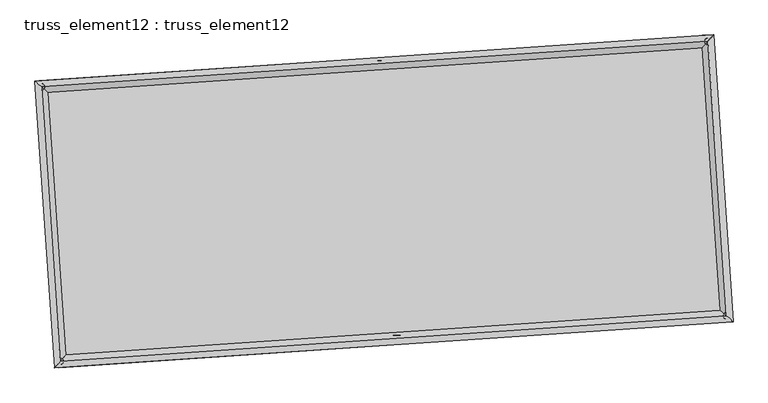
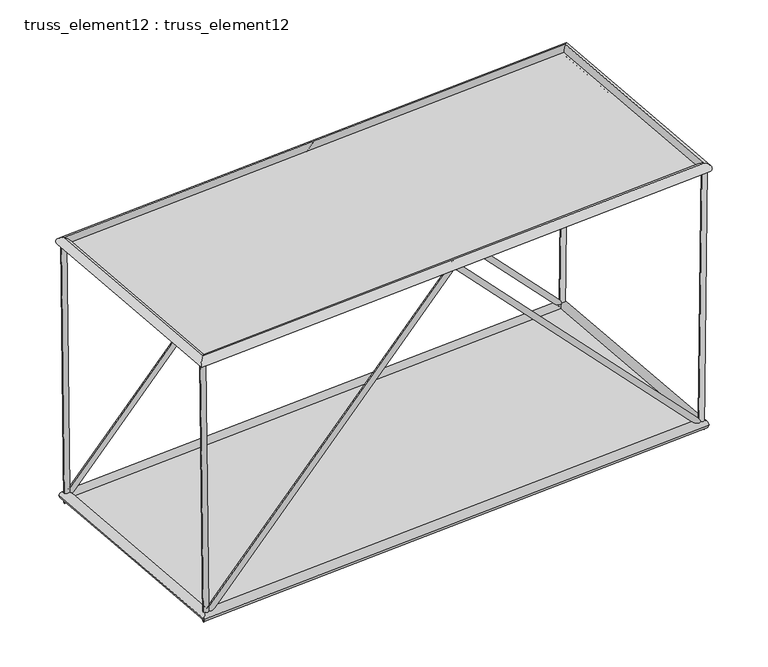
"""IFC4 building model written with IfcOpenShell, lengths in millimetres: plate geometry, truss_element12 : truss_element12."""

from ifc_helpers import new_model, si_unit, frame, origin, origin_with_axes, place, context, project, spatial, polyline, circle_curve, ellipse_curve, outline, extrude, source, transform, mapped, element, save
from ifc_brep_helpers import plane_surface, cylinder_surface, advanced_brep


def truss_element12_truss_element12_d70bcacd(model_context):
    return source(origin(), model_context, "Body", "SolidModel", [
        advanced_brep(
        [(-3725.0104614, 2272.1281216, 5000.2382654), (-3824.1066063, 2258.7673379, 4999.0367904), (-3666.4119315, 2276.1237326, 122.6729842), (-3762.5749513, 2262.9629475, -122.6729842), (1063.1790008, 2598.6165594, 5071.765221), (1063.6352741, 2592.0438766, 4927.5226673), (5793.8246657, 2921.1813044, 122.680509), (5890.9363113, 2921.1991841, -122.680509), (5851.3764049, 2925.1055388, 5000.2403686), (5951.3692127, 2925.3198739, 4999.0603521)],
        [
            (0, 1, circle_curve(frame((-3774.5585339, 2265.4477297, 4999.6375279), z_axis=(-0.012013018486842605, -0.0008191220648593599, 0.9999275055852188), x_axis=(-0.1336079931124214, 0.9910339423186926, -0.0007933150329807116)), 50.0)),
            (1, 0, circle_curve(frame((-3774.5585339, 2265.4477297, 4999.6375279), z_axis=(-0.012013018486842605, -0.0008191220648593599, 0.9999275055852188), x_axis=(-0.1336079931124214, 0.9910339423186926, -0.0007933150329807116)), 50.0)),
            (0, 2),
            (2, 3, ellipse_curve(frame((-3714.4934414, 2269.54334, 0.0), z_axis=(-0.9280153260656253, -0.06327783736789783, 0.3671286830055), x_axis=(0.366278191257424, 0.02497511750808738, 0.9301701619137474)), 132.1694786, 50.0)),
            (3, 1),
            (3, 2, ellipse_curve(frame((-3714.4934414, 2269.54334, 0.0), z_axis=(-0.9280153260656253, -0.06327783736789783, 0.3671286830055), x_axis=(0.366278191257424, 0.02497511750808738, 0.9301701619137474)), 132.1694786, 50.0)),
            (2, 4),
            (4, 5, ellipse_curve(frame((1063.4071375, 2595.330218, 4999.6439441), z_axis=(-0.9976833945063722, -0.06802823812175049, -5.607399430392597e-05), x_axis=(5.5944093068511954e-05, 3.8146150427985738e-06, -0.9999999984278536)), 72.2783214, 50.0)),
            (5, 3),
            (5, 4, ellipse_curve(frame((1063.4071375, 2595.330218, 4999.6439441), z_axis=(-0.9976833945063722, -0.06802823812175049, -5.607399430392597e-05), x_axis=(5.5944093068511954e-05, 3.8146150427985738e-06, -0.9999999984278536)), 72.2783214, 50.0)),
            (4, 6),
            (6, 7, ellipse_curve(frame((5842.3804885, 2921.1902443, 0.0), z_axis=(-0.9279553876166273, -0.06327375039290756, -0.3672808613370581), x_axis=(-0.36643001705206174, -0.024985469931879827, 0.9301100842886872)), 132.1861236, 50.0)),
            (7, 5),
            (7, 6, ellipse_curve(frame((5842.3804885, 2921.1902443, 0.0), z_axis=(-0.9279553876166273, -0.06327375039290756, -0.3672808613370581), x_axis=(-0.36643001705206174, -0.024985469931879827, 0.9301100842886872)), 132.1861236, 50.0)),
            (8, 9, circle_curve(frame((5901.3728088, 2925.2127063, 4999.6503604), z_axis=(0.011798464054869244, 0.0008044924137406994, 0.9999300720739939), x_axis=(-0.002152694612337802, 0.9999973794150412, -0.0007791462995799872)), 50.0)),
            (9, 8, circle_curve(frame((5901.3728088, 2925.2127063, 4999.6503604), z_axis=(0.011798464054869244, 0.0008044924137406994, 0.9999300720739939), x_axis=(-0.002152694612337802, 0.9999973794150412, -0.0007791462995799872)), 50.0)),
            (6, 8),
            (9, 7),
        ],
        [
            plane_surface(frame((-3774.5585339, 2315.4477129, 4999.678487), z_axis=(-0.012013018486842117, -0.0008191220648596661, 0.9999275055852188), x_axis=(0.9999278410899632, -9.840838612440448e-06, 0.012013014456126566))),
            cylinder_surface(frame((-3774.5585339, 2265.4477297, 4999.6375279), z_axis=(-0.012013018486842605, -0.0008191220648593599, 0.9999275055852188), x_axis=(-0.1336079931124214, 0.9910339423186926, -0.0007933150329807116)), 50.0),
            cylinder_surface(frame((-3714.4934414, 2269.54334, 0.0), z_axis=(-0.6901273969450528, -0.04705716377784427, -0.7221563537926055), x_axis=(-0.020411408362793253, 0.9987523871322667, -0.0455745938681458)), 50.0),
            cylinder_surface(frame((1063.4071375, 2595.330218, 4999.6439441), z_axis=(-0.690208193369534, -0.04706267297889348, 0.7220787731388079), x_axis=(-0.11534434850610661, 0.9922792708177843, -0.04557992949783976)), 50.0),
            plane_surface(frame((5901.3728088, 2875.2127225, 4999.6905878), z_axis=(0.011798464054869178, 0.0008044924137361026, 0.9999300720739939), x_axis=(0.9999303957005938, -9.49243553982625e-06, -0.011798460236306582))),
            cylinder_surface(frame((5842.3804885, 2921.1902443, 0.0), z_axis=(-0.011798464054869241, -0.0008044924137406992, -0.9999300720739936), x_axis=(-0.002152694612337802, 0.9999973794150412, -0.0007791462995799872)), 50.0),
        ],
        [
            (0, [[1, 2]]),
            (1, [[-1, 3, 4, 5]]),
            (1, [[-2, -5, 6, -3]]),
            (2, [[-4, 7, 8, 9]]),
            (2, [[-6, -9, 10, -7]]),
            (3, [[-8, 11, 12, 13]]),
            (3, [[-10, -13, 14, -11]]),
            (4, [[15, 16]]),
            (5, [[-12, 17, -16, 18]]),
            (5, [[-14, -18, -15, -17]]),
        ],
    ),
        advanced_brep(
        [(-3452.8975085, -1718.6054627, 5000.2382654), (-3551.9936533, -1731.9662464, 4999.0367904), (-3394.2989786, -1714.6098517, 122.6729842), (-3490.4619984, -1727.7706368, -122.6729842), (1335.2919537, -1392.1170249, 5071.765221), (1335.748227, -1398.6897077, 4927.5226673), (6065.9376186, -1069.5522799, 122.680509), (6163.0492642, -1069.5344002, -122.680509), (6123.4893578, -1065.6280455, 5000.2403686), (6223.4821656, -1065.4137104, 4999.0603521)],
        [
            (0, 1, circle_curve(frame((-3502.4455809, -1725.2858546, 4999.6375279), z_axis=(-0.01201301848684304, -0.0008191220648593858, 0.9999275055852187), x_axis=(-0.13360799311242097, 0.9910339423186927, -0.000793315032980739)), 50.0)),
            (1, 0, circle_curve(frame((-3502.4455809, -1725.2858546, 4999.6375279), z_axis=(-0.01201301848684304, -0.0008191220648593858, 0.9999275055852187), x_axis=(-0.13360799311242097, 0.9910339423186927, -0.000793315032980739)), 50.0)),
            (0, 2),
            (2, 3, ellipse_curve(frame((-3442.3804885, -1721.1902443, 0.0), z_axis=(-0.9280153260656255, -0.06327783736789769, 0.36712868300549933), x_axis=(0.3662781912574234, 0.02497511750808728, 0.9301701619137478)), 132.1694786, 50.0)),
            (3, 1),
            (3, 2, ellipse_curve(frame((-3442.3804885, -1721.1902443, 0.0), z_axis=(-0.9280153260656255, -0.06327783736789769, 0.36712868300549933), x_axis=(0.3662781912574234, 0.02497511750808728, 0.9301701619137478)), 132.1694786, 50.0)),
            (2, 4),
            (4, 5, ellipse_curve(frame((1335.5200904, -1395.4033663, 4999.6439441), z_axis=(-0.9976833945063722, -0.06802823812175042, -5.607399430400622e-05), x_axis=(5.594409306866568e-05, 3.8146150429042725e-06, -0.9999999984278536)), 72.2783214, 50.0)),
            (5, 3),
            (5, 4, ellipse_curve(frame((1335.5200904, -1395.4033663, 4999.6439441), z_axis=(-0.9976833945063722, -0.06802823812175042, -5.607399430400622e-05), x_axis=(5.594409306866568e-05, 3.8146150429042725e-06, -0.9999999984278536)), 72.2783214, 50.0)),
            (4, 6),
            (6, 7, ellipse_curve(frame((6114.4934414, -1069.54334, 0.0), z_axis=(-0.9279553876166274, -0.0632737503929075, -0.3672808613370576), x_axis=(-0.36643001705206135, -0.024985469931879837, 0.9301100842886875)), 132.1861236, 50.0)),
            (7, 5),
            (7, 6, ellipse_curve(frame((6114.4934414, -1069.54334, 0.0), z_axis=(-0.9279553876166274, -0.0632737503929075, -0.3672808613370576), x_axis=(-0.36643001705206135, -0.024985469931879837, 0.9301100842886875)), 132.1861236, 50.0)),
            (8, 9, circle_curve(frame((6173.4857617, -1065.520878, 4999.6503604), z_axis=(0.011798464054869687, 0.0008044924137406689, 0.9999300720739938), x_axis=(-0.0021526946123380866, 0.9999973794150413, -0.0007791462995799525)), 50.0)),
            (9, 8, circle_curve(frame((6173.4857617, -1065.520878, 4999.6503604), z_axis=(0.011798464054869687, 0.0008044924137406689, 0.9999300720739938), x_axis=(-0.0021526946123380866, 0.9999973794150413, -0.0007791462995799525)), 50.0)),
            (6, 8),
            (9, 7),
        ],
        [
            plane_surface(frame((-3502.4455809, -1675.2858714, 4999.678487), z_axis=(-0.012013018486842117, -0.000819122064859655, 0.9999275055852188), x_axis=(0.9999278410899632, -9.840838612440448e-06, 0.012013014456126566))),
            cylinder_surface(frame((-3502.4455809, -1725.2858546, 4999.6375279), z_axis=(-0.012013018486843044, -0.000819122064859386, 0.9999275055852189), x_axis=(-0.13360799311242097, 0.9910339423186927, -0.000793315032980739)), 50.0),
            cylinder_surface(frame((-3442.3804885, -1721.1902443, 0.0), z_axis=(-0.6901273969450527, -0.04705716377784414, -0.7221563537926058), x_axis=(-0.020411408362793246, 0.9987523871322667, -0.045574593868145614)), 50.0),
            cylinder_surface(frame((1335.5200904, -1395.4033663, 4999.6439441), z_axis=(-0.6902081933695338, -0.04706267297889348, 0.7220787731388081), x_axis=(-0.1153443485061065, 0.9922792708177844, -0.04557992949783957)), 50.0),
            plane_surface(frame((6173.4857617, -1115.5208618, 4999.6905878), z_axis=(0.01179846405486918, 0.0008044924137360949, 0.9999300720739939), x_axis=(0.9999303957005938, -9.49243554027034e-06, -0.011798460236306582))),
            cylinder_surface(frame((6114.4934414, -1069.54334, 0.0), z_axis=(-0.011798464054869687, -0.0008044924137406689, -0.9999300720739938), x_axis=(-0.0021526946123380866, 0.9999973794150413, -0.0007791462995799525)), 50.0),
        ],
        [
            (0, [[1, 2]]),
            (1, [[-1, 3, 4, 5]]),
            (1, [[-2, -5, 6, -3]]),
            (2, [[-4, 7, 8, 9]]),
            (2, [[-6, -9, 10, -7]]),
            (3, [[-8, 11, 12, 13]]),
            (3, [[-10, -13, 14, -11]]),
            (4, [[15, 16]]),
            (5, [[-12, 17, -16, 18]]),
            (5, [[-14, -18, -15, -17]]),
        ],
    ),
        advanced_brep(
        [(-3502.4422112, -1725.2821197, 4909.637528), (-3502.4489507, -1725.2895894, 5089.6375279), (-3774.5623794, 2265.4509726, 5089.6375279), (-3774.5546883, 2265.4444869, 4909.637528), (5901.3759409, 2925.216425, 5089.6503603), (5901.3696766, 2925.2089877, 4909.6503604), (6173.4893696, -1065.524137, 5089.6503603), (6173.4821538, -1065.5176189, 4909.6503604)],
        [
            (0, 1, ellipse_curve(frame((-3502.4455809, -1725.2858546, 4999.6375279), z_axis=(-0.7535719234048375, 0.6573654662781263, -9.356088951893453e-07), x_axis=(-0.6573654662774667, -0.7535719234054129, -9.356088948066304e-07)), 127.2792206, 90.0)),
            (1, 2),
            (2, 3, ellipse_curve(frame((-3774.5585339, 2265.4477297, 4999.6375279), z_axis=(-0.6573654662774665, -0.7535719234054131, -9.356088948857094e-07), x_axis=(0.7535719234048378, -0.657365466278126, 9.356088952684248e-07)), 127.2792206, 90.0)),
            (3, 0),
            (1, 0, ellipse_curve(frame((-3502.4455809, -1725.2858546, 4999.6375279), z_axis=(-0.7535719234048375, 0.6573654662781263, -9.356088951893453e-07), x_axis=(-0.6573654662774667, -0.7535719234054129, -9.356088948066304e-07)), 127.2792206, 90.0)),
            (3, 2, ellipse_curve(frame((-3774.5585339, 2265.4477297, 4999.6375279), z_axis=(-0.6573654662774665, -0.7535719234054131, -9.356088948857094e-07), x_axis=(0.7535719234048378, -0.657365466278126, 9.356088952684248e-07)), 127.2792206, 90.0)),
            (2, 4),
            (4, 5, ellipse_curve(frame((5901.3728088, 2925.2127063, 4999.6503604), z_axis=(-0.7535719234048375, 0.6573654662781261, -9.356088950771271e-07), x_axis=(-0.6573654662774668, -0.7535719234054126, -9.356088950770072e-07)), 127.2792206, 90.0)),
            (5, 3),
            (5, 4, ellipse_curve(frame((5901.3728088, 2925.2127063, 4999.6503604), z_axis=(-0.7535719234048375, 0.6573654662781261, -9.356088950771271e-07), x_axis=(-0.6573654662774668, -0.7535719234054126, -9.356088950770072e-07)), 127.2792206, 90.0)),
            (4, 6),
            (6, 7, ellipse_curve(frame((6173.4857617, -1065.520878, 4999.6503604), z_axis=(0.6573654662774666, 0.7535719234054129, 9.356088949979278e-07), x_axis=(-0.7535719234048374, 0.6573654662781263, -9.356088949980478e-07)), 127.2792206, 90.0)),
            (7, 5),
            (7, 6, ellipse_curve(frame((6173.4857617, -1065.520878, 4999.6503604), z_axis=(0.6573654662774666, 0.7535719234054129, 9.356088949979278e-07), x_axis=(-0.7535719234048374, 0.6573654662781263, -9.356088949980478e-07)), 127.2792206, 90.0)),
            (6, 1),
            (0, 7),
        ],
        [
            cylinder_surface(frame((-3502.4455809, -1725.2858546, 4999.6375279), z_axis=(0.06802823822869676, -0.997683396074877, 0.0), x_axis=(-0.9976833952696054, -0.06802823817378835, -4.017813848481856e-05)), 90.0),
            cylinder_surface(frame((-3774.5585339, 2265.4477297, 4999.6375279), z_axis=(-0.9976833960740037, -0.06802823822863736, -1.3231507884948943e-06), x_axis=(-0.06802823812605353, 0.9976833953252681, -3.8854987697593246e-05)), 90.0),
            cylinder_surface(frame((5901.3728088, 2925.2127063, 4999.6503604), z_axis=(-0.06802823822869698, 0.9976833960748769, 0.0), x_axis=(0.9976833953721892, 0.06802823818078337, -3.753183691009722e-05)), 90.0),
            cylinder_surface(frame((6173.4857617, -1065.520878, 4999.6503604), z_axis=(0.9976833960740037, 0.06802823822863724, 1.3231507883830595e-06), x_axis=(0.06802823822863723, -0.9976833953182733, -3.885498769748157e-05)), 90.0),
        ],
        [
            (0, [[1, 2, 3, 4]]),
            (0, [[5, -4, 6, -2]]),
            (1, [[-3, 7, 8, 9]]),
            (1, [[-6, -9, 10, -7]]),
            (2, [[-8, 11, 12, 13]]),
            (2, [[-10, -13, 14, -11]]),
            (3, [[-12, 15, -1, 16]]),
            (3, [[-14, -16, -5, -15]]),
        ],
    ),
        advanced_brep(
        [(-3358.7115243, -1625.2761972, 0.0), (-3526.0494527, -1817.1042913, 0.0), (-3810.4074885, 2353.2123043, 0.0), (-3618.5793943, 2185.8743758, 0.0), (5926.0494527, 3017.1042913, 0.0), (5758.7115243, 2825.2761972, 0.0), (6210.4074885, -1153.2123043, 0.0), (6018.5793943, -985.8743758, 0.0)],
        [
            (0, 1, ellipse_curve(frame((-3442.3804885, -1721.1902443, 0.0), z_axis=(-0.7535719234054578, 0.657365466278081, 0.0), x_axis=(-0.657365466278081, -0.7535719234054578, 0.0)), 127.2792206, 90.0)),
            (1, 2),
            (2, 3, ellipse_curve(frame((-3714.4934414, 2269.54334, 0.0), z_axis=(-0.6573654662780809, -0.753571923405458, 0.0), x_axis=(0.753571923405458, -0.6573654662780807, 0.0)), 127.2792206, 90.0)),
            (3, 0),
            (1, 0, ellipse_curve(frame((-3442.3804885, -1721.1902443, 0.0), z_axis=(-0.7535719234054578, 0.657365466278081, 0.0), x_axis=(-0.657365466278081, -0.7535719234054578, 0.0)), 127.2792206, 90.0)),
            (3, 2, ellipse_curve(frame((-3714.4934414, 2269.54334, 0.0), z_axis=(-0.6573654662780809, -0.753571923405458, 0.0), x_axis=(0.753571923405458, -0.6573654662780807, 0.0)), 127.2792206, 90.0)),
            (2, 4),
            (4, 5, ellipse_curve(frame((5842.3804885, 2921.1902443, 0.0), z_axis=(-0.7535719234054578, 0.657365466278081, 0.0), x_axis=(-0.657365466278081, -0.7535719234054578, 0.0)), 127.2792206, 90.0)),
            (5, 3),
            (5, 4, ellipse_curve(frame((5842.3804885, 2921.1902443, 0.0), z_axis=(-0.7535719234054578, 0.657365466278081, 0.0), x_axis=(-0.657365466278081, -0.7535719234054578, 0.0)), 127.2792206, 90.0)),
            (4, 6),
            (6, 7, ellipse_curve(frame((6114.4934414, -1069.54334, 0.0), z_axis=(0.6573654662780812, 0.7535719234054576, 0.0), x_axis=(-0.7535719234054576, 0.6573654662780812, 0.0)), 127.2792206, 90.0)),
            (7, 5),
            (7, 6, ellipse_curve(frame((6114.4934414, -1069.54334, 0.0), z_axis=(0.6573654662780812, 0.7535719234054576, 0.0), x_axis=(-0.7535719234054576, 0.6573654662780812, 0.0)), 127.2792206, 90.0)),
            (6, 1),
            (0, 7),
        ],
        [
            cylinder_surface(frame((-3442.3804885, -1721.1902443, 0.0), z_axis=(0.06802823822870128, -0.9976833960748767, 0.0), x_axis=(-0.9976833960748767, -0.06802823822870128, 0.0)), 90.0),
            cylinder_surface(frame((-3714.4934414, 2269.54334, 0.0), z_axis=(-0.9976833960748767, -0.06802823822870108, 0.0), x_axis=(-0.06802823822870108, 0.9976833960748767, 0.0)), 90.0),
            cylinder_surface(frame((5842.3804885, 2921.1902443, 0.0), z_axis=(-0.0680282382287008, 0.9976833960748767, 0.0), x_axis=(0.9976833960748767, 0.0680282382287008, 0.0)), 90.0),
            cylinder_surface(frame((6114.4934414, -1069.54334, 0.0), z_axis=(0.9976833960748767, 0.06802823822870059, 0.0), x_axis=(0.06802823822870059, -0.9976833960748767, 0.0)), 90.0),
        ],
        [
            (0, [[1, 2, 3, 4]]),
            (0, [[5, -4, 6, -2]]),
            (1, [[-3, 7, 8, 9]]),
            (1, [[-6, -9, 10, -7]]),
            (2, [[-8, 11, 12, 13]]),
            (2, [[-10, -13, 14, -11]]),
            (3, [[-12, 15, -1, 16]]),
            (3, [[-14, -16, -5, -15]]),
        ],
    ),
        extrude(outline(polyline([(-3442.3804885, -1721.1902443), (-3714.4934414, 2269.54334), (5842.3804885, 2921.1902443), (6114.4934414, -1069.54334), (-3442.3804885, -1721.1902443)])), origin_with_axes(), (0.0, 0.0, 1.0), 20.0),
        extrude(outline(polyline([(-2000.0000001, 4849.1993455), (1999.9999999, 4849.1993456), (1999.9999999, -4849.1993456), (-2000.0, -4849.1993456), (-2000.0000001, 4849.1993455)])), frame((1199.4636139, 599.9634259, 4999.6439441), z_axis=(-1.3200855722030626e-06, -9.001161678212776e-08, 0.9999999999991247), x_axis=(-0.0680282382287005, 0.9976833960748767, 0.0)), (0.0, 0.0, 1.0), 20.0),
    ])


if __name__ == "__main__":
    model = new_model("IFC4")
    model_context = context("Model", 3, world=origin())
    ifc_project = project(units=[si_unit("LENGTHUNIT", "METRE", prefix="MILLI")], contexts=[model_context])
    site = spatial("IfcSite", under=ifc_project)
    building = spatial("IfcBuilding", under=site)
    placement = place(None, origin())
    truss_element12_truss_element12_shape = truss_element12_truss_element12_d70bcacd(model_context)
    element("IfcPlate", 1, ObjectType="truss_element12 : truss_element12", at=placement, inside=building, context=model_context, shape_type="MappedRepresentation", body=[
        mapped(truss_element12_truss_element12_shape, transform((0.0, 0.0, 0.0), x_axis=(1.0, 0.0, 0.0), y_axis=(0.0, 1.0, 0.0), z_axis=(0.0, 0.0, 1.0))),
    ])
    save(model, "model.ifc")

# Revit data of these elements
# Type "truss_element12 : truss_element12"
#   steellbar1 = 90 mm
#   steelbar2 = 50 mm
#   offset1 = 5000 mm
#   M = Default Roof
# Element 1 (IfcPlate, "truss_element12 : truss_element12")
#   Materials on its faces: "Default Roof"
# Materials
#   "Default Roof": class "Miscellaneous", colour RGB 0 127 0, transparency 0, Comments = "Rendering appearance not upgraded Rendering appearance not upgraded ", Cost = 0
